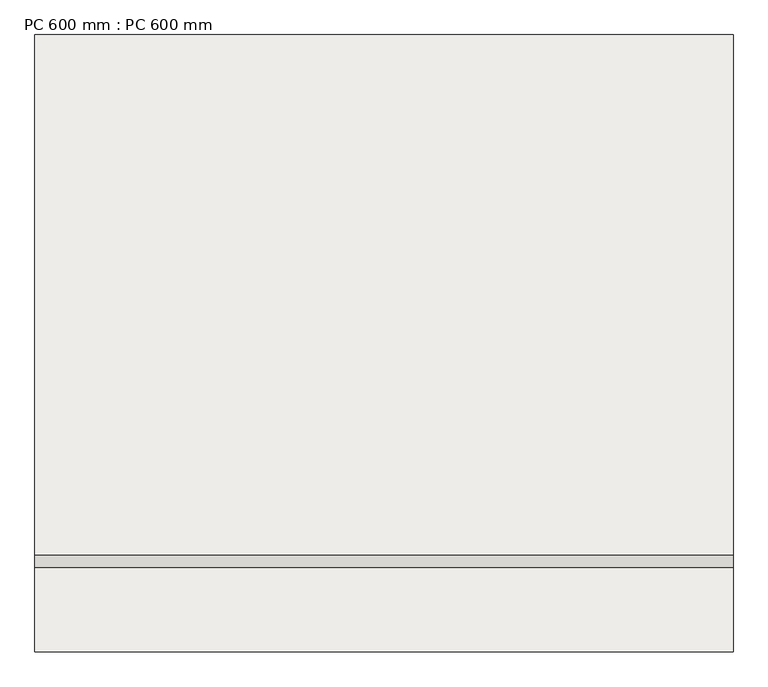
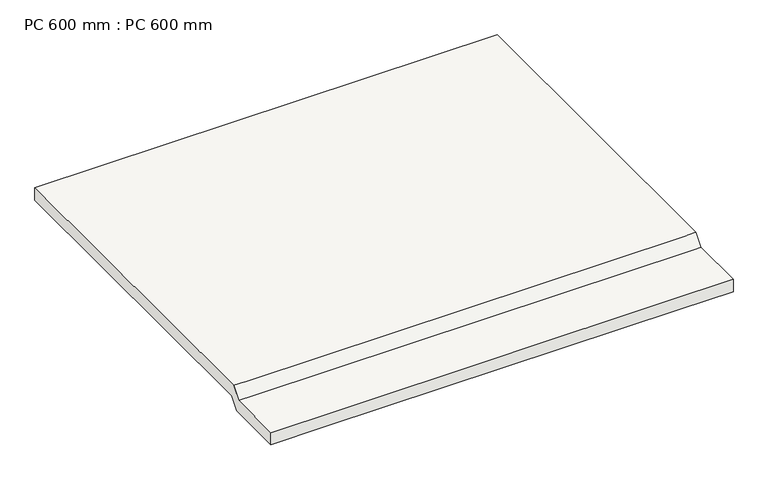
"""IFC4 building model written with IfcOpenShell, lengths in millimetres: slab geometry, PC 600 mm : PC 600 mm."""

from ifc_helpers import new_model, si_unit, origin, place, context, project, spatial, faceted_brep, source, transform, mapped, element, save


def pc_600_mm_pc_600_mm_16fd50b2(model_context):
    return source(origin(), model_context, "Body", "Brep", [
        faceted_brep([(20800.0, 25300.0, -6120.0), (20800.0, 9209.5951826, -6120.0), (20800.0, 8809.6095449, -6619.9808175), (20800.0, 6200.0, -6619.9808175), (20800.0, 6200.0, -7220.0), (20800.0, 8953.7810717, -7220.0), (20800.0, 9353.7820554, -6720.0), (20800.0, 25300.0, -6720.0), (-800.0, 25300.0, -6120.0), (-800.0, 25300.0, -6720.0), (-800.0, 9353.7820554, -6720.0), (-800.0, 8953.7810717, -7220.0), (-800.0, 6200.0, -7220.0), (-800.0, 6200.0, -6619.9808175), (-800.0, 8809.6095449, -6619.9808175), (-800.0, 9209.5951826, -6120.0), (-200.0, 9209.5951826, -6120.0), (20200.0, 9209.5951826, -6120.0), (-200.0, 8809.6095449, -6619.9808175), (20200.0, 8809.6095449, -6619.9808175), (2300.0, 6200.0, -6619.9808175), (17700.0, 6200.0, -6619.9808175), (1700.0, 6200.0, -7220.0), (18300.0, 6200.0, -7220.0)], [[[0, 1, 2, 3, 4, 5, 6, 7]], [[8, 9, 10, 11, 12, 13, 14, 15]], [[1, 0, 8, 15, 16, 17]], [[2, 1, 17, 16, 15, 14, 18, 19]], [[3, 2, 19, 18, 14, 13, 20, 21]], [[4, 3, 21, 20, 13, 12, 22, 23]], [[5, 4, 23, 22, 12, 11]], [[6, 5, 11, 10]], [[7, 6, 10, 9]], [[0, 7, 9, 8]]]),
    ])


if __name__ == "__main__":
    model = new_model("IFC4")
    model_context = context("Model", 3, world=origin())
    ifc_project = project(units=[si_unit("LENGTHUNIT", "METRE", prefix="MILLI")], contexts=[model_context])
    site = spatial("IfcSite", under=ifc_project)
    building = spatial("IfcBuilding", under=site)
    placement = place(None, origin())
    pc_600_mm_pc_600_mm_shape = pc_600_mm_pc_600_mm_16fd50b2(model_context)
    element("IfcSlab", 1, ObjectType="PC 600 mm : PC 600 mm", at=placement, inside=building, context=model_context, shape_type="MappedRepresentation", body=[
        mapped(pc_600_mm_pc_600_mm_shape, transform((0.0, 0.0, 0.0), x_axis=(1.0, 0.0, 0.0), y_axis=(0.0, 1.0, 0.0), z_axis=(0.0, 0.0, 1.0))),
    ])
    save(model, "model.ifc")

# Revit data of these elements
# Project information
#   Project Issue Date = "Issue Date"
#   Project Status = "Project Status"
#   Client Name = "Owner"
#   Project Address = "Enter address here"
#   Project Name = "Project Name"
#   Project Number = "Project Number"
# Type "PC 600 mm : PC 600 mm"
#   Structural Material = Concrete, PC
# Element 1 (IfcSlab, "PC 600 mm : PC 600 mm")
#   Materials on its faces: "Concrete, PC"
# Materials
#   "Concrete, PC": class "Concrete", colour RGB 162 162 162, transparency 0, Description = "Concrete slab topping", Cost = 0
